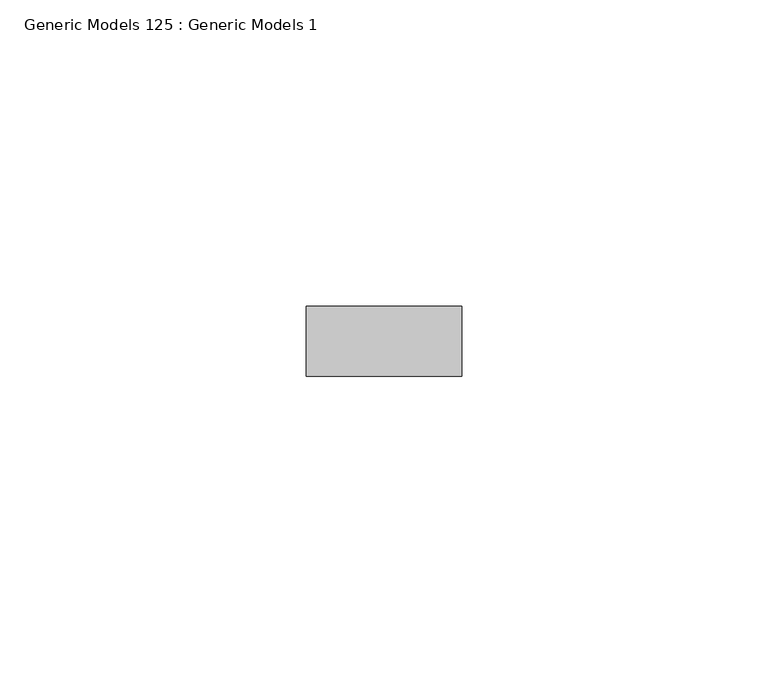
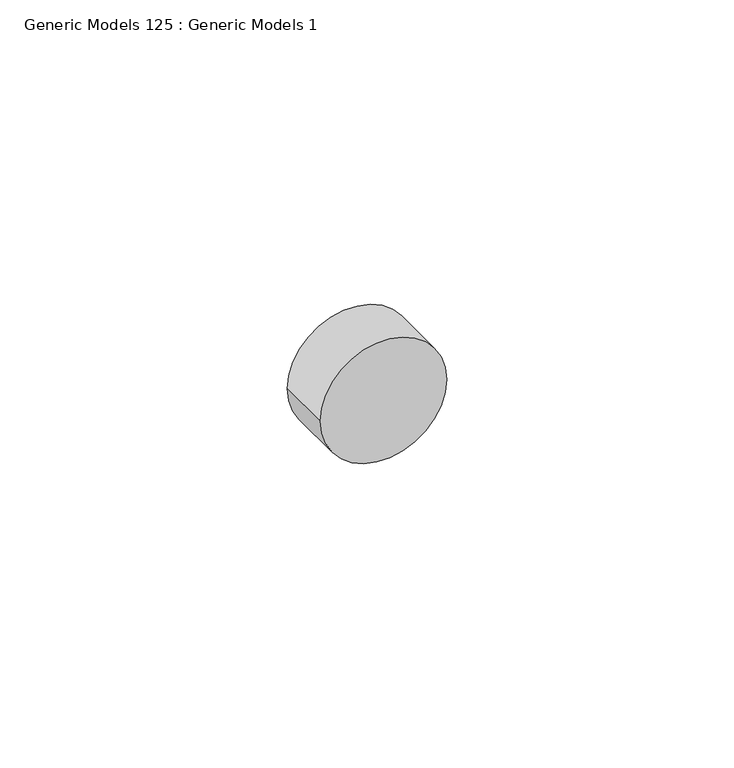
"""IFC4 building model written with IfcOpenShell, lengths in millimetres: proxy geometry, Generic Models 125 : Generic Models 1."""

import ifcopenshell
import ifcopenshell.guid

model = None  # the IFC model being written
_history = None  # IfcOwnerHistory: only IFC2X3 demands one
_inside = {}  # id of a spatial element -> (the spatial element, [elements in it])
_under = {}  # id of a project, library or spatial element -> (it, [spatial elements below it])
_declared = {}  # id of a project -> (the project, [libraries it declares])
_typed = {}  # id of a type object -> (the type object, [elements of that type])
_made_of = {}  # id of a material, layer set ... -> (it, [elements and type objects made of it])


def new_model(schema):
    """Start an empty IFC model of exactly this schema.

    Asked for "IFC4X3", IfcOpenShell would pick the latest addendum, in which some entities
    have other attributes; the version numbers below select the first issue.
    IFC2X3 requires an IfcOwnerHistory on every rooted entity: one is made here for all.
    """
    global model, _history
    if schema == "IFC4X3":
        model = ifcopenshell.file(schema_version=(4, 3, 0, 0))
    else:
        model = ifcopenshell.file(schema=schema)
    _inside.clear()
    _under.clear()
    _declared.clear()
    _typed.clear()
    _made_of.clear()
    _history = None
    if model.schema == "IFC2X3":
        org = make("IfcOrganization", Name="unknown")
        user = make(
            "IfcPersonAndOrganization",
            ThePerson=make("IfcPerson", FamilyName="unknown"),
            TheOrganization=org,
        )
        app = make(
            "IfcApplication",
            ApplicationDeveloper=org,
            Version="unknown",
            ApplicationFullName="unknown",
            ApplicationIdentifier="unknown",
        )
        _history = make(
            "IfcOwnerHistory",
            OwningUser=user,
            OwningApplication=app,
            ChangeAction="ADDED",
            CreationDate=0,
        )
    return model


def make(cls, **values):
    """One entity of the class cls with the attributes given. An attribute that is None is left unset."""
    return model.create_entity(
        cls, **{name: value for name, value in values.items() if value is not None}
    )


def rooted(cls, **values):
    """An entity with a GlobalId (a new one), such as an element, a storey or a relation."""
    return make(cls, GlobalId=ifcopenshell.guid.new(), OwnerHistory=_history, **values)


def si_unit(unit_type, name, prefix=None):
    """IfcSIUnit, for example si_unit("LENGTHUNIT", "METRE", prefix="MILLI")."""
    return make("IfcSIUnit", UnitType=unit_type, Prefix=prefix, Name=name)


def assignment(units):
    """IfcUnitAssignment: the units of a project."""
    return None if units is None else make("IfcUnitAssignment", Units=units)


def point(xyz):
    """IfcCartesianPoint."""
    return None if xyz is None else make("IfcCartesianPoint", Coordinates=xyz)


def direction(xyz):
    """IfcDirection."""
    return None if xyz is None else make("IfcDirection", DirectionRatios=xyz)


def frame(location, z_axis=None, x_axis=None):
    """IfcAxis2Placement3D, a coordinate frame: its origin and axes. An axis left out is left unset."""
    return make(
        "IfcAxis2Placement3D",
        Location=point(location),
        Axis=direction(z_axis),
        RefDirection=direction(x_axis),
    )


def frame_2d(location, x_axis=None):
    """IfcAxis2Placement2D, a coordinate frame in the plane: its origin and x axis."""
    return make(
        "IfcAxis2Placement2D", Location=point(location), RefDirection=direction(x_axis)
    )


def origin():
    """The frame at (0, 0, 0) with its axes left unset."""
    return frame((0.0, 0.0, 0.0))


def place(relative_to, where):
    """IfcLocalPlacement: puts the frame where relative to a parent placement (None: the world)."""
    return make(
        "IfcLocalPlacement", PlacementRelTo=relative_to, RelativePlacement=where
    )


def context(
    kind, dimensions, precision=None, world=None, true_north=None, identifier=None
):
    """IfcGeometricRepresentationContext, for example the 3D "Model" context."""
    return make(
        "IfcGeometricRepresentationContext",
        ContextIdentifier=identifier,
        ContextType=kind,
        CoordinateSpaceDimension=dimensions,
        Precision=precision,
        WorldCoordinateSystem=world,
        TrueNorth=true_north,
    )


def project(units=None, contexts=None):
    """IfcProject with its units and contexts."""
    return rooted(
        "IfcProject",
        Name="project",
        RepresentationContexts=contexts,
        UnitsInContext=assignment(units),
    )


def spatial(cls, under=None, at=None, **own):
    """A site, building, storey or space (cls), placed at a placement, below another one or the project."""
    s = rooted(cls, ObjectPlacement=at, **own)
    if under is not None:
        _under.setdefault(under.id(), (under, []))[1].append(s)
    return s


def circle_curve(where, radius):
    """IfcCircle in the frame where."""
    return make("IfcCircle", Position=where, Radius=radius)


def trimmed(basis, trim1, trim2, sense, master):
    """IfcTrimmedCurve: the piece of a basis curve between two trims."""
    return make(
        "IfcTrimmedCurve",
        BasisCurve=basis,
        Trim1=trim1,
        Trim2=trim2,
        SenseAgreement=sense,
        MasterRepresentation=master,
    )


def segment(curve, same_sense, transition):
    """IfcCompositeCurveSegment."""
    return make(
        "IfcCompositeCurveSegment",
        Transition=transition,
        SameSense=same_sense,
        ParentCurve=curve,
    )


def composite_curve(segments, self_intersect=None):
    """IfcCompositeCurve: segments joined end to end."""
    return make("IfcCompositeCurve", Segments=segments, SelfIntersect=self_intersect)


def outline(outer, holes=None, kind="AREA"):
    """IfcArbitraryClosedProfileDef: a profile drawn as a closed curve; with holes, ...WithVoids."""
    if holes is None:
        return make("IfcArbitraryClosedProfileDef", ProfileType=kind, OuterCurve=outer)
    return make(
        "IfcArbitraryProfileDefWithVoids",
        ProfileType=kind,
        OuterCurve=outer,
        InnerCurves=holes,
    )


def extrude(swept, where, along, depth):
    """IfcExtrudedAreaSolid: the profile swept, set in the frame where, extruded along a direction by depth."""
    return make(
        "IfcExtrudedAreaSolid",
        SweptArea=swept,
        Position=where,
        ExtrudedDirection=direction(along),
        Depth=depth,
    )


def shape(context_of_items, identifier, shape_type, items):
    """IfcShapeRepresentation: the items that make up one representation, for example the "Body"."""
    return make(
        "IfcShapeRepresentation",
        ContextOfItems=context_of_items,
        RepresentationIdentifier=identifier,
        RepresentationType=shape_type,
        Items=items,
    )


def source(mapping_origin, context_of_items, identifier, shape_type, items):
    """IfcRepresentationMap: a shape defined once, which mapped items show again and again."""
    return make(
        "IfcRepresentationMap",
        MappingOrigin=mapping_origin,
        MappedRepresentation=shape(context_of_items, identifier, shape_type, items),
    )


def transform(
    local_origin,
    x_axis=None,
    y_axis=None,
    z_axis=None,
    scale=None,
    scale2=None,
    scale3=None,
    uniform=True,
):
    """IfcCartesianTransformationOperator3D, or its non-uniform kind. x_axis, y_axis, z_axis: its Axis1, 2, 3."""
    if uniform:
        return make(
            "IfcCartesianTransformationOperator3D",
            Axis1=direction(x_axis),
            Axis2=direction(y_axis),
            LocalOrigin=point(local_origin),
            Scale=scale,
            Axis3=direction(z_axis),
        )
    return make(
        "IfcCartesianTransformationOperator3DnonUniform",
        Axis1=direction(x_axis),
        Axis2=direction(y_axis),
        LocalOrigin=point(local_origin),
        Scale=scale,
        Axis3=direction(z_axis),
        Scale2=scale2,
        Scale3=scale3,
    )


def mapped(mapping_source, mapping_target):
    """IfcMappedItem: shows the shape of a source again, moved by a transform."""
    return make(
        "IfcMappedItem", MappingSource=mapping_source, MappingTarget=mapping_target
    )


def made_of(thing, what):
    """Note that an element or type object is made of a material, layer set ...; save() writes the relation."""
    if what is not None:
        _made_of.setdefault(what.id(), (what, []))[1].append(thing)
    return thing


def element(
    cls,
    number,
    at=None,
    inside=None,
    cuts=None,
    type_object=None,
    material=None,
    context=None,
    identifier="Body",
    shape_type=None,
    held_by="IfcProductDefinitionShape",
    body=None,
    shapes=None,
    **own,
):
    """One element of the class cls, such as IfcWall. Its Tag is "e" and its number.

    at: its placement. inside: the storey or other place that contains it. cuts: it is an
    opening in that element (IfcRelVoidsElement). A single representation is given by context,
    identifier, shape_type and body (its items); several are given by shapes. held_by: the class
    of the entity that holds the representations. save() writes the other relations.
    """
    e = rooted(cls, Tag="e%d" % number, ObjectPlacement=at, **own)
    if body is not None:
        shapes = [shape(context, identifier, shape_type, body)]
    if shapes is not None:
        e.Representation = make(held_by, Representations=shapes)
    if inside is not None:
        _inside.setdefault(inside.id(), (inside, []))[1].append(e)
    if cuts is not None:
        rooted(
            "IfcRelVoidsElement", RelatingBuildingElement=cuts, RelatedOpeningElement=e
        )
    if type_object is not None:
        _typed.setdefault(type_object.id(), (type_object, []))[1].append(e)
    return made_of(e, material)


def aggregate(whole, parts):
    """IfcRelAggregates: a whole, such as a stair, and the parts it consists of."""
    return rooted("IfcRelAggregates", RelatingObject=whole, RelatedObjects=parts)


def save(model, path):
    """Write the relations noted so far, then the file.

    IfcRelAggregates (storeys below a building ...), IfcRelContainedInSpatialStructure (elements
    in a storey), IfcRelDefinesByType, IfcRelAssociatesMaterial and IfcRelDeclares: one each for
    every whole, place, type object, material and project.
    """
    for whole, parts in _under.values():
        aggregate(whole, parts)
    for where, things in _inside.values():
        rooted(
            "IfcRelContainedInSpatialStructure",
            RelatedElements=things,
            RelatingStructure=where,
        )
    for kind, things in _typed.values():
        rooted("IfcRelDefinesByType", RelatedObjects=things, RelatingType=kind)
    for what, things in _made_of.values():
        rooted("IfcRelAssociatesMaterial", RelatedObjects=things, RelatingMaterial=what)
    for by, libraries in _declared.values():
        rooted("IfcRelDeclares", RelatingContext=by, RelatedDefinitions=libraries)
    model.write(path)


def generic_models_125_generic_models_1_a24d3eef(model_context):
    return source(origin(), model_context, "Body", "SweptSolid", [
        extrude(outline(composite_curve([segment(trimmed(circle_curve(frame_2d((38374.9548538, 7686.9828124)), 12.7), [point((38374.9548538, 7674.2828124))], [point((38374.9548538, 7699.6828124))], False, "CARTESIAN"), True, "CONTINUOUS"), segment(trimmed(circle_curve(frame_2d((38374.9548538, 7686.9828124)), 12.7), [point((38374.9548538, 7699.6828124))], [point((38374.9548538, 7674.2828124))], False, "CARTESIAN"), True, "CONTINUOUS")], self_intersect=False)), frame((0.0, 1836.9202358, 0.0), z_axis=(0.0, 1.0, 0.0), x_axis=(0.0, 0.0, 1.0)), (0.0, 0.0, 1.0), 11.4464372),
    ])


if __name__ == "__main__":
    model = new_model("IFC4")
    model_context = context("Model", 3, world=origin())
    ifc_project = project(units=[si_unit("LENGTHUNIT", "METRE", prefix="MILLI")], contexts=[model_context])
    site = spatial("IfcSite", under=ifc_project)
    building = spatial("IfcBuilding", under=site)
    placement = place(None, origin())
    generic_models_125_generic_models_1_shape = generic_models_125_generic_models_1_a24d3eef(model_context)
    element("IfcBuildingElementProxy", 1, Name="Generic Models 125 : Generic Models 1", ObjectType="Generic Models 125 : Generic Models 1", at=placement, inside=building, context=model_context, shape_type="MappedRepresentation", body=[
        mapped(generic_models_125_generic_models_1_shape, transform((0.0, 0.0, 0.0), x_axis=(1.0, 0.0, 0.0), y_axis=(0.0, 1.0, 0.0), z_axis=(0.0, 0.0, 1.0))),
    ])
    save(model, "model.ifc")

# Revit data of these elements
# Element 1 (IfcBuildingElementProxy, "Generic Models 125 : Generic Models 1")
#   Materials on its faces: "S.S. LAG BOLT - SEE STRUCT. DWGS"
# Materials
#   "S.S. LAG BOLT - SEE STRUCT. DWGS": class "Generic", colour RGB 120 120 120, transparency 0, Cost = 0
